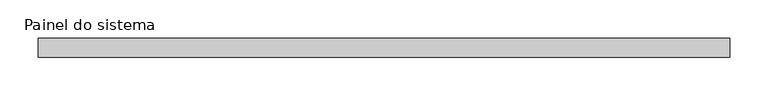
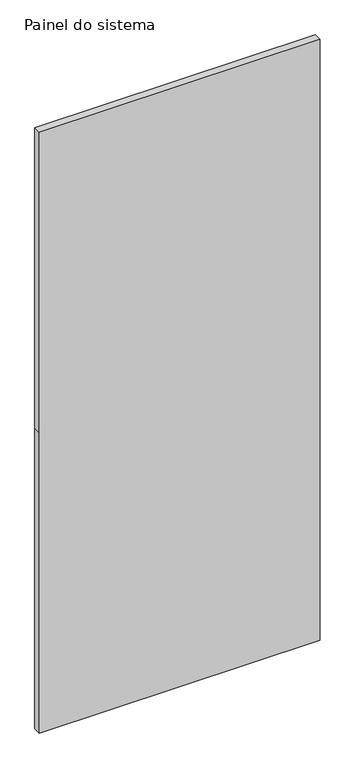
"""IFC4 building model written with IfcOpenShell, lengths in millimetres: plate geometry, Painel do sistema : Envidraçado."""

from ifc_helpers import new_model, si_unit, frame, origin, place, context, project, spatial, polyline, outline, extrude, source, transform, mapped, element, save


def painel_do_sistema_78d5b6fe(model_context):
    return source(origin(), model_context, "Body", "SweptSolid", [
        extrude(outline(polyline([(0.0, -453.0083333), (0.0, 453.0083333), (1025.0, 453.0083333), (2050.0, 453.0083333), (2050.0, -453.0083333), (1025.0, -453.0083333), (0.0, -453.0083333)])), frame((0.0, 24.5, 0.0), z_axis=(0.0, 1.0, 0.0), x_axis=(0.0, 0.0, 1.0)), (0.0, 0.0, 1.0), 25.0),
    ])


if __name__ == "__main__":
    model = new_model("IFC4")
    model_context = context("Model", 3, world=origin())
    ifc_project = project(units=[si_unit("LENGTHUNIT", "METRE", prefix="MILLI")], contexts=[model_context])
    site = spatial("IfcSite", under=ifc_project)
    building = spatial("IfcBuilding", under=site)
    placement = place(None, origin())
    painel_do_sistema_shape = painel_do_sistema_78d5b6fe(model_context)
    element("IfcPlate", 1, ObjectType="Painel do sistema : Envidraçado", at=placement, inside=building, context=model_context, shape_type="MappedRepresentation", body=[
        mapped(painel_do_sistema_shape, transform((0.0, 0.0, 0.0), x_axis=(1.0, 0.0, 0.0), y_axis=(0.0, 1.0, 0.0), z_axis=(0.0, 0.0, 1.0))),
    ])
    save(model, "model.ifc")

# Revit data of these elements
# Type "Painel do sistema : Envidraçado"
#   Construction Type Id = "GSP4R"
#   Analytic Construction = "Vidraça única Pilkington 1/8 pol"
#   Visual Light Transmittance = 0.9
#   Solar Heat Gain Coefficient = 0.86
#   Heat Transfer Coefficient (U) = 6.7069 W/(m²·K)
# Element 1 (IfcPlate, "Painel do sistema : Envidraçado")
#   Materials on its faces: ".VIDRO GENÉRICO"
# Materials
#   ".VIDRO GENÉRICO": class ".CC_VIDRO", colour RGB 0 128 192, transparency 0.9, Description = "Vidro comum", Cost = 0
